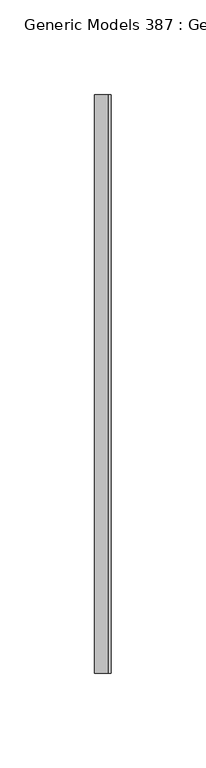
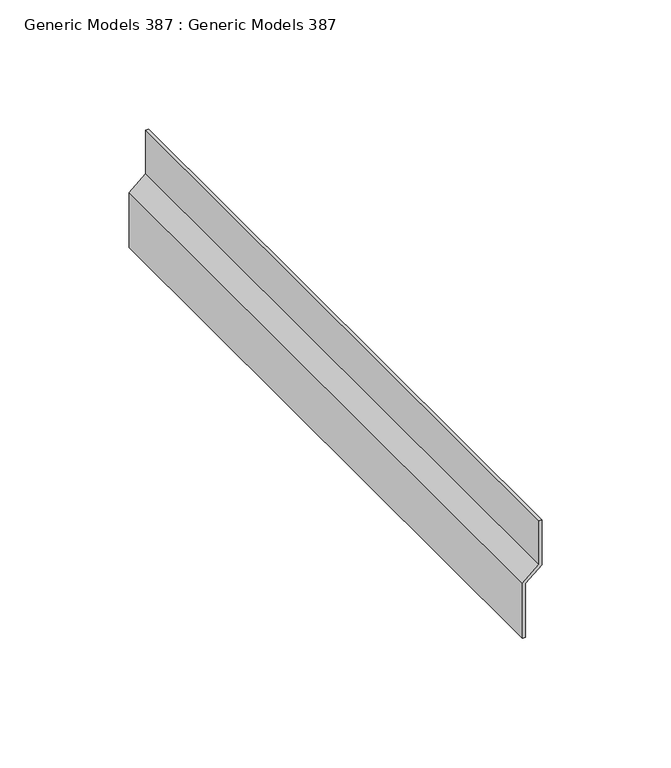
"""IFC4 building model written with IfcOpenShell, lengths in millimetres: proxy geometry, Generic Models 387 : Generic Models 387."""

from ifc_helpers import new_model, si_unit, frame, origin, place, context, project, spatial, polyline, outline, extrude, source, transform, mapped, element, save


def generic_models_387_generic_models_387_bf171670(model_context):
    return source(origin(), model_context, "Body", "SweptSolid", [
        extrude(outline(polyline([(129066.5864185, -7109.7860419), (129072.8222791, -7102.3544325), (129094.1393732, -7102.3544325), (129094.1393732, -7103.6442763), (129073.4237431, -7103.6442763), (129067.1878825, -7111.0758856), (129041.0275266, -7111.0758856), (129041.0275266, -7109.7860419), (129066.5864185, -7109.7860419)])), frame((0.0, -4250.542257, 0.0), z_axis=(0.0, 1.0, 0.0), x_axis=(0.0, 0.0, 1.0)), (0.0, 0.0, 1.0), 304.8),
    ])


if __name__ == "__main__":
    model = new_model("IFC4")
    model_context = context("Model", 3, world=origin())
    ifc_project = project(units=[si_unit("LENGTHUNIT", "METRE", prefix="MILLI")], contexts=[model_context])
    site = spatial("IfcSite", under=ifc_project)
    building = spatial("IfcBuilding", under=site)
    placement = place(None, origin())
    generic_models_387_generic_models_387_shape = generic_models_387_generic_models_387_bf171670(model_context)
    element("IfcBuildingElementProxy", 1, Name="Generic Models 387 : Generic Models 387", ObjectType="Generic Models 387 : Generic Models 387", at=placement, inside=building, context=model_context, shape_type="MappedRepresentation", body=[
        mapped(generic_models_387_generic_models_387_shape, transform((0.0, 0.0, 0.0), x_axis=(1.0, 0.0, 0.0), y_axis=(0.0, 1.0, 0.0), z_axis=(0.0, 0.0, 1.0))),
    ])
    save(model, "model.ifc")
